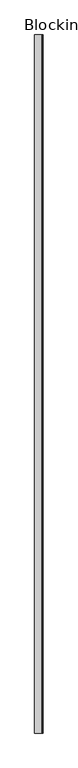
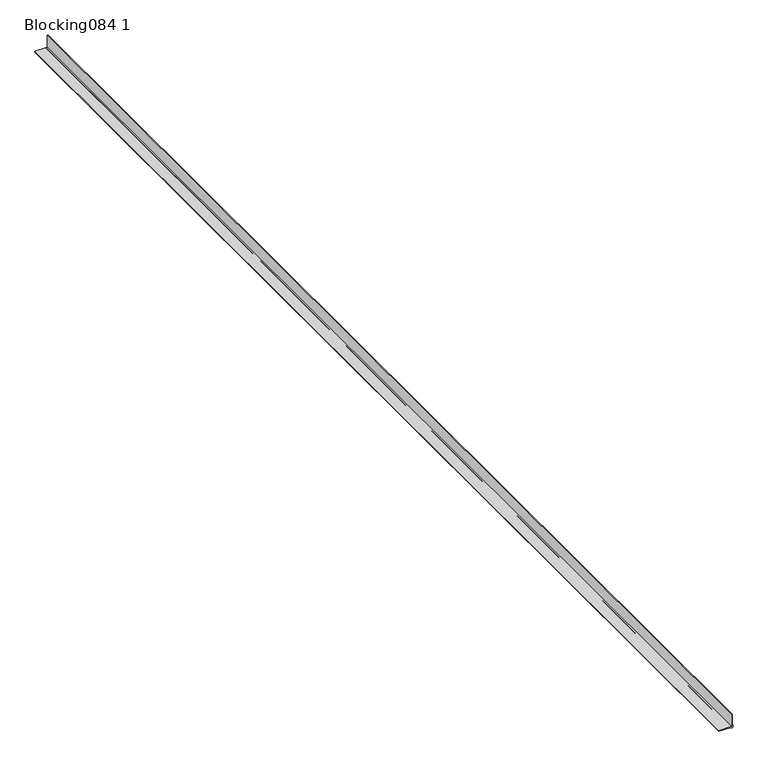
"""IFC4 building model written with IfcOpenShell, lengths in millimetres: proxy geometry, Blocking084 1 : Blocking084 10484."""

from ifc_helpers import new_model, si_unit, point, frame, frame_2d, origin, place, context, project, spatial, polyline, circle_curve, trimmed, segment, composite_curve, outline, extrude, source, transform, mapped, element, save


def blocking084_1_7f017c89(model_context):
    return source(origin(), model_context, "Body", "SweptSolid", [
        extrude(outline(composite_curve([segment(polyline([(42121.2158547, 6211.4587308), (42100.0626708, 6211.4587308), (42100.0626708, 6190.3055469), (42098.7826708, 6190.3055469), (42098.7826708, 6209.1570759)]), True, "CONTINUOUS"), segment(trimmed(circle_curve(frame_2d((42100.0626708, 6211.4587308)), 2.6336316), [point((42098.7826708, 6209.1570759))], [point((42102.3643257, 6212.7387308))], False, "CARTESIAN"), True, "CONTINUOUS"), segment(polyline([(42102.3643257, 6212.7387308), (42121.2158547, 6212.7387308), (42121.2158547, 6211.4587308)]), True, "CONTINUOUS")], self_intersect=False)), frame((0.0, -1052.8912362, 0.0), z_axis=(0.0, 1.0, 0.0), x_axis=(0.0, 0.0, 1.0)), (0.0, 0.0, 1.0), 2000.0),
    ])


if __name__ == "__main__":
    model = new_model("IFC4")
    model_context = context("Model", 3, world=origin())
    ifc_project = project(units=[si_unit("LENGTHUNIT", "METRE", prefix="MILLI")], contexts=[model_context])
    site = spatial("IfcSite", under=ifc_project)
    building = spatial("IfcBuilding", under=site)
    placement = place(None, origin())
    blocking084_1_shape = blocking084_1_7f017c89(model_context)
    element("IfcBuildingElementProxy", 1, Name="Blocking084 1 : Blocking084 10484", ObjectType="Blocking084 1 : Blocking084 10484", at=placement, inside=building, context=model_context, shape_type="MappedRepresentation", body=[
        mapped(blocking084_1_shape, transform((0.0, 0.0, 0.0), x_axis=(1.0, 0.0, 0.0), y_axis=(0.0, 1.0, 0.0), z_axis=(0.0, 0.0, 1.0))),
    ])
    save(model, "model.ifc")

# Revit data of these elements
# Type "Blocking084 1 : Blocking084 10484"
#   NameOverride = "Blocking084"
# Element 1 (IfcBuildingElementProxy, "Blocking084 1 : Blocking084 10484")
#   Materials on its faces: "CORNER BEAD"
# Materials
#   "CORNER BEAD": class "Unassigned", colour RGB 253 236 176, transparency 0, Cost = 0
